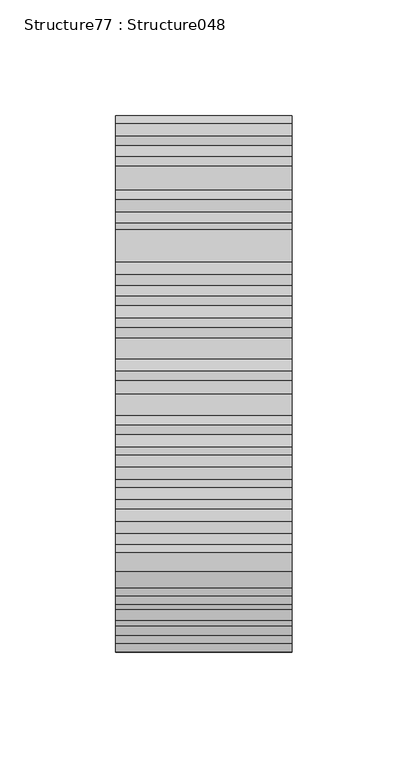
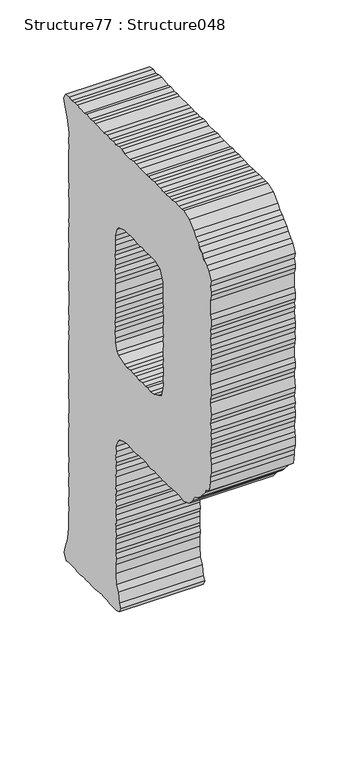
"""IFC4 building model written with IfcOpenShell, lengths in millimetres: proxy geometry, Structure77 : Structure048."""

from ifc_helpers import new_model, si_unit, frame, origin, place, context, project, spatial, polyline, outline, extrude, source, transform, mapped, element, save


def structure77_structure048_e401d336(model_context):
    return source(origin(), model_context, "Body", "SweptSolid", [
        extrude(outline(polyline([(278339.7895607, 3996.390138), (278348.592421, 3996.390138), (278353.2730523, 3997.5486624), (278357.3728168, 3997.5486624), (278362.6551748, 3996.390138), (278366.7565439, 3996.9645864), (278371.4355706, 3996.390138), (278376.1386664, 3996.9645864), (278381.3985599, 3996.390138), (278395.4597091, 3996.390138), (278398.4025538, 3996.9645864), (278403.0815805, 3996.390138), (278408.341474, 3997.5486624), (278412.4653076, 3996.390138), (278423.0059545, 3997.5486624), (278427.1073236, 3997.5486624), (278431.7863503, 3996.390138), (278435.8877194, 3997.5486624), (278441.1700774, 3996.9645864), (278444.6681152, 3991.6806238), (278442.9303285, 3986.4046842), (278441.1700774, 3982.8793681), (278439.9874839, 3978.2035506), (278438.2272327, 3973.5197101), (278435.8877194, 3962.9774586), (278437.0687083, 3954.7506513), (278435.8877194, 3948.917914), (278437.0687083, 3944.8165449), (278437.0687083, 3935.4328178), (278436.4669816, 3931.3346579), (278436.4669816, 3921.3748778), (278437.0687083, 3917.2735087), (278435.8877194, 3912.0071968), (278436.4669816, 3906.7328618), (278436.4669816, 3903.2059411), (278435.8877194, 3898.5301236), (278435.8877194, 3883.2863809), (278436.4669816, 3879.1769888), (278435.8877194, 3875.0772243), (278437.0687083, 3870.4030114), (278436.4669816, 3864.5446004), (278437.0687083, 3860.4432313), (278435.8877194, 3855.1769193), (278436.4669816, 3851.0595042), (278436.4669816, 3832.8921721), (278435.8877194, 3828.2163546), (278435.8877194, 3823.5341187), (278436.4669816, 3818.8310229), (278437.0687083, 3812.9726119), (278435.8877194, 3808.8888934), (278435.8877194, 3800.0876378), (278436.4669816, 3794.2292268), (278437.0687083, 3790.7039107), (278435.8877194, 3786.0280932), (278437.0687083, 3780.1616592), (278435.8877194, 3776.0618947), (278437.0687083, 3771.3860772), (278435.8877194, 3766.684586), (278436.4669816, 3762.0023501), (278436.4669816, 3756.7440611), (278437.0687083, 3752.6170184), (278437.0687083, 3743.2332913), (278436.4669816, 3739.1592005), (278437.0687083, 3733.8736333), (278435.8877194, 3729.7738688), (278436.4669816, 3723.9154578), (278436.4669816, 3720.4158154), (278437.0687083, 3715.1302482), (278436.4669816, 3709.8559132), (278435.8877194, 3705.7545441), (278435.8877194, 3696.9709391), (278436.4669816, 3691.0868544), (278436.4669816, 3686.4030139), (278435.8877194, 3682.8857208), (278436.4669816, 3678.2018803), (278437.0687083, 3672.9435914), (278436.4669816, 3668.8261762), (278436.4669816, 3662.9854159), (278437.0687083, 3658.3015753), (278437.0687083, 3654.1841602), (278435.8877194, 3650.1004418), (278437.0687083, 3644.2420307), (278436.4669816, 3639.5405396), (278435.8877194, 3635.4407751), (278436.4669816, 3630.7392839), (278436.4669816, 3626.6571701), (278435.8877194, 3620.7971545), (278435.8877194, 3616.0972679), (278437.0687083, 3612.0135494), (278437.0687083, 3607.8961343), (278435.8877194, 3602.6298224), (278437.0687083, 3597.9540049), (278437.0687083, 3593.8285667), (278436.4669816, 3588.5702778), (278436.4669816, 3584.4689087), (278438.2272327, 3573.9266571), (278438.8289594, 3570.4109687), (278441.1700774, 3564.54293), (278442.9303285, 3559.8671125), (278444.088853, 3556.3417965), (278440.5683507, 3550.4833855), (278436.4669816, 3551.0658569), (278426.5055969, 3551.0658569), (278423.0059545, 3550.4833855), (278418.3044633, 3550.4833855), (278413.0445698, 3551.0658569), (278408.341474, 3550.4833855), (278404.2417095, 3551.0658569), (278399.5610782, 3550.4833855), (278395.4597091, 3550.4833855), (278384.9190622, 3551.6675836), (278381.3985599, 3551.6675836), (278377.2971908, 3551.0658569), (278372.0372973, 3550.4833855), (278362.0534481, 3550.4833855), (278357.3728168, 3551.6675836), (278355.0333035, 3556.3417965), (278357.3728168, 3559.8671125), (278359.1346725, 3569.2524442), (278362.0534481, 3575.0851816), (278363.234437, 3584.4689087), (278363.234437, 3593.2541183), (278362.0534481, 3599.1125293), (278363.234437, 3603.7963698), (278362.6551748, 3607.3393366), (278363.234437, 3613.1720739), (278363.234437, 3617.8559144), (278362.0534481, 3621.3732075), (278363.234437, 3626.6571701), (278362.6551748, 3630.7392839), (278362.0534481, 3636.0408972), (278363.234437, 3640.7167147), (278363.234437, 3645.9830266), (278362.0534481, 3649.5003197), (278362.6551748, 3654.7842823), (278362.6551748, 3659.4584952), (278362.0534481, 3664.1423357), (278362.6551748, 3668.8261762), (278362.6551748, 3677.6274319), (278362.0534481, 3683.4858429), (278363.234437, 3687.587212), (278362.0534481, 3691.6869765), (278362.6551748, 3696.3884676), (278362.0534481, 3702.229228), (278363.234437, 3706.3289925), (278359.7139348, 3713.9556777), (278357.3728168, 3716.8985223), (278349.7734099, 3719.2316172), (278343.8909298, 3720.4158154), (278339.2102985, 3719.8140887), (278335.1089294, 3719.8140887), (278331.0091649, 3719.2316172), (278325.7268069, 3720.4158154), (278316.9464111, 3720.4158154), (278311.0847909, 3719.8140887), (278307.5642887, 3719.2316172), (278302.3043951, 3720.4158154), (278298.203026, 3719.8140887), (278292.3430104, 3719.8140887), (278288.8209035, 3719.2316172), (278284.1402722, 3719.8140887), (278279.4387811, 3719.2316172), (278274.7581497, 3720.4158154), (278264.796765, 3720.4158154), (278259.5368715, 3719.8140887), (278256.0163692, 3719.2316172), (278247.8152357, 3722.1568112), (278243.7138666, 3726.8566978), (278237.8522463, 3733.8736333), (278233.1732196, 3736.2163558), (278230.230375, 3739.1592005), (278223.1877659, 3747.3587295), (278220.8482525, 3750.8583719), (278216.1676212, 3753.2171405), (278214.4073701, 3762.5848215), (278214.4073701, 3767.2590344), (278213.2488456, 3771.9605256), (278213.2488456, 3780.1616592), (278213.8281078, 3784.8438951), (278214.4073701, 3790.1294623), (278213.8281078, 3795.4037973), (278213.2488456, 3799.5051664), (278213.2488456, 3804.1890069), (278213.8281078, 3808.8888934), (278213.2488456, 3812.9726119), (278214.4073701, 3818.8310229), (278213.8281078, 3822.348316), (278213.2488456, 3827.6162325), (278214.4073701, 3838.1761347), (278214.4073701, 3841.6741725), (278213.2488456, 3846.3772683), (278213.2488456, 3851.6612309), (278214.4073701, 3856.3161885), (278214.4073701, 3865.7015202), (278213.8281078, 3869.8189354), (278213.2488456, 3874.5043805), (278213.8281078, 3880.3627915), (278213.2488456, 3885.0626781), (278213.2488456, 3889.7208449), (278213.8281078, 3893.822214), (278214.4073701, 3899.7046941), (278213.8281078, 3904.3901392), (278214.4073701, 3908.46423), (278213.2488456, 3912.5896682), (278213.2488456, 3918.4480792), (278214.4073701, 3923.1319197), (278214.4073701, 3936.6186205), (278213.2488456, 3941.8753048), (278213.2488456, 3945.4182716), (278214.4073701, 3950.6765605), (278213.2488456, 3955.9348494), (278216.7468834, 3963.5615346), (278220.2689903, 3966.5043792), (278224.3687548, 3970.5768654), (278226.7098727, 3974.1214368), (278231.3888994, 3977.6194746), (278233.7300174, 3980.5623192), (278237.2729841, 3983.4794902), (278240.7726265, 3987.5792547), (278247.8152357, 3994.0233463), (278256.0163692, 3997.5486624), (278259.5368715, 3996.9645864), (278264.2175028, 3996.9645864), (278269.4773964, 3997.5486624), (278274.7581497, 3996.9645864), (278278.8595188, 3996.9645864), (278284.1402722, 3996.390138), (278287.6399146, 3996.390138), (278292.9222726, 3996.9645864), (278298.203026, 3996.9645864), (278301.7026684, 3997.5486624), (278306.9850264, 3996.390138), (278311.0847909, 3997.5486624), (278315.18616, 3996.390138), (278324.5682825, 3996.390138), (278330.4299027, 3996.9645864), (278334.5296672, 3997.5486624), (278339.7895607, 3996.390138)]), holes=[polyline([(278357.952079, 3797.1463977), (278360.3156615, 3799.5051664), (278363.234437, 3805.9476534), (278363.234437, 3810.6298893), (278363.8136993, 3816.4883003), (278363.234437, 3821.1737455), (278363.8136993, 3824.7167122), (278362.6551748, 3829.9733965), (278363.234437, 3834.0474873), (278362.6551748, 3839.3587282), (278363.234437, 3844.6154125), (278362.6551748, 3848.1166595), (278363.234437, 3853.4198774), (278363.234437, 3862.8036045), (278362.6551748, 3867.4601667), (278362.6551748, 3871.5599312), (278363.8136993, 3876.263027), (278363.234437, 3880.3627915), (278362.6551748, 3886.2051565), (278363.8136993, 3889.7208449), (278362.6551748, 3894.4030808), (278362.6551748, 3899.7046941), (278363.234437, 3904.3901392), (278362.6551748, 3909.0627475), (278360.8949237, 3916.0909152), (278357.952079, 3919.6066036), (278349.1716832, 3922.5494483), (278334.5296672, 3922.5494483), (278329.828176, 3921.9733953), (278326.3285336, 3921.3748778), (278321.0461756, 3922.5494483), (278316.9464111, 3921.3748778), (278311.0847909, 3921.9733953), (278301.7026684, 3921.9733953), (278294.0807971, 3919.0321552), (278292.3430104, 3915.5068392), (278289.4226302, 3909.0627475), (278288.8209035, 3904.3901392), (278289.4226302, 3900.2887701), (278288.8209035, 3895.0048075), (278289.4226302, 3889.7208449), (278288.2416413, 3886.2051565), (278289.4226302, 3880.9452629), (278288.2416413, 3876.263027), (278288.2416413, 3870.9790644), (278288.8209035, 3866.3032469), (278288.8209035, 3862.2018778), (278288.2416413, 3857.5019912), (278289.4226302, 3854.0007442), (278288.2416413, 3848.7167816), (278289.4226302, 3844.0345457), (278288.8209035, 3839.3587282), (278288.2416413, 3835.2332901), (278288.8209035, 3830.5574726), (278288.2416413, 3825.849563), (278288.2416413, 3821.1737455), (278289.4226302, 3816.4883003), (278288.2416413, 3810.6298893), (278289.4226302, 3807.1045732), (278291.1604169, 3798.9050443), (278295.261786, 3797.1463977), (278302.3043951, 3793.6451507), (278307.5642887, 3793.0723069), (278312.2657798, 3793.6451507), (278315.7878867, 3793.0723069), (278320.4669134, 3793.6451507), (278325.7268069, 3793.0723069), (278331.0091649, 3793.6451507), (278334.5296672, 3793.6451507), (278339.2102985, 3794.2292268), (278344.4926565, 3793.6451507), (278348.592421, 3794.2292268), (278357.952079, 3797.1463977)])]), frame((-59031.6926606, 0.0, 0.0), z_axis=(1.0, 0.0, 0.0), x_axis=(0.0, 1.0, 0.0)), (0.0, 0.0, 1.0), 76.2),
    ])


if __name__ == "__main__":
    model = new_model("IFC4")
    model_context = context("Model", 3, world=origin())
    ifc_project = project(units=[si_unit("LENGTHUNIT", "METRE", prefix="MILLI")], contexts=[model_context])
    site = spatial("IfcSite", under=ifc_project)
    building = spatial("IfcBuilding", under=site)
    placement = place(None, origin())
    structure77_structure048_shape = structure77_structure048_e401d336(model_context)
    element("IfcBuildingElementProxy", 1, Name="Structure77 : Structure048", ObjectType="Structure77 : Structure048", at=placement, inside=building, context=model_context, shape_type="MappedRepresentation", body=[
        mapped(structure77_structure048_shape, transform((0.0, 0.0, 0.0), x_axis=(1.0, 0.0, 0.0), y_axis=(0.0, 1.0, 0.0), z_axis=(0.0, 0.0, 1.0))),
    ])
    save(model, "model.ifc")

# Revit data of these elements
# Type "Structure77 : Structure048"
#   NameOverride = "Structure048"
# Element 1 (IfcBuildingElementProxy, "Structure77 : Structure048")
#   Materials on its faces: "BRUSHED ALUM. LETTERING"
# Materials
#   "BRUSHED ALUM. LETTERING": class "Unassigned", colour RGB 169 181 186, transparency 0, Cost = 0
